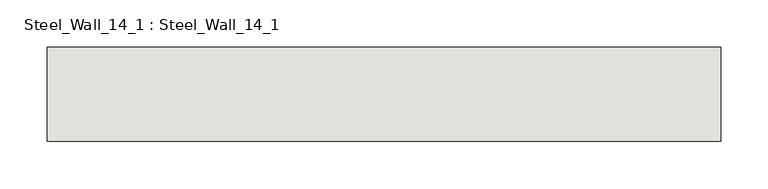
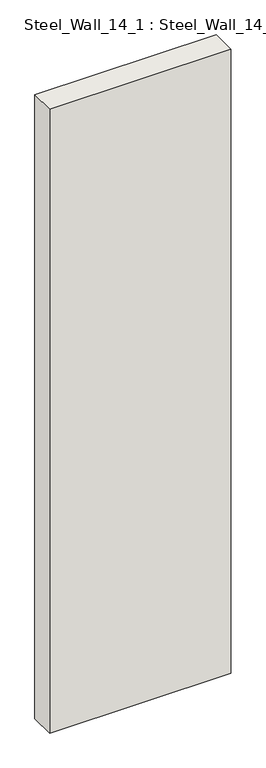
"""IFC4 building model written with IfcOpenShell, lengths in millimetres: wall geometry, Steel_Wall_14_1 : Steel_Wall_14_1."""

from ifc_helpers import new_model, si_unit, frame, origin, place, context, project, spatial, polyline, outline, extrude, source, transform, mapped, element, save


def steel_wall_14_1_steel_wall_14_1_bad66547(model_context):
    return source(origin(), model_context, "Body", "SweptSolid", [
        extrude(outline(polyline([(930.0, 395.0), (215.0, 395.0), (215.0, 495.0), (930.0, 495.0), (930.0, 395.0)])), frame((0.0, 0.0, 250.0), z_axis=(0.0, 0.0, 1.0), x_axis=(1.0, 0.0, 0.0)), (0.0, 0.0, 1.0), 2600.0),
    ])


if __name__ == "__main__":
    model = new_model("IFC4")
    model_context = context("Model", 3, world=origin())
    ifc_project = project(units=[si_unit("LENGTHUNIT", "METRE", prefix="MILLI")], contexts=[model_context])
    site = spatial("IfcSite", under=ifc_project)
    building = spatial("IfcBuilding", under=site)
    placement = place(None, origin())
    steel_wall_14_1_steel_wall_14_1_shape = steel_wall_14_1_steel_wall_14_1_bad66547(model_context)
    element("IfcWall", 1, ObjectType="Steel_Wall_14_1 : Steel_Wall_14_1", at=placement, inside=building, context=model_context, shape_type="MappedRepresentation", body=[
        mapped(steel_wall_14_1_steel_wall_14_1_shape, transform((0.0, 0.0, 0.0), x_axis=(1.0, 0.0, 0.0), y_axis=(0.0, 1.0, 0.0), z_axis=(0.0, 0.0, 1.0))),
    ])
    save(model, "model.ifc")

# Revit data of these elements
# Type "Steel_Wall_14_1 : Steel_Wall_14_1"
#   NameOverride = "Steel_Wall_14_1"
# Element 1 (IfcWall, "Steel_Wall_14_1 : Steel_Wall_14_1")
#   Materials on its faces: "IfcSurfaceStyle #33"
# Materials
#   "IfcSurfaceStyle #33": class "Unassigned", colour RGB 214 214 214, transparency 0
